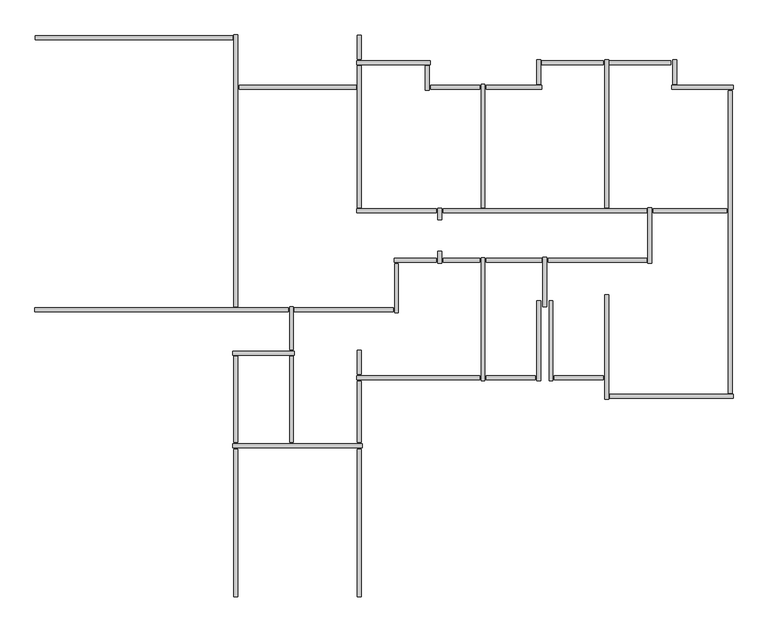
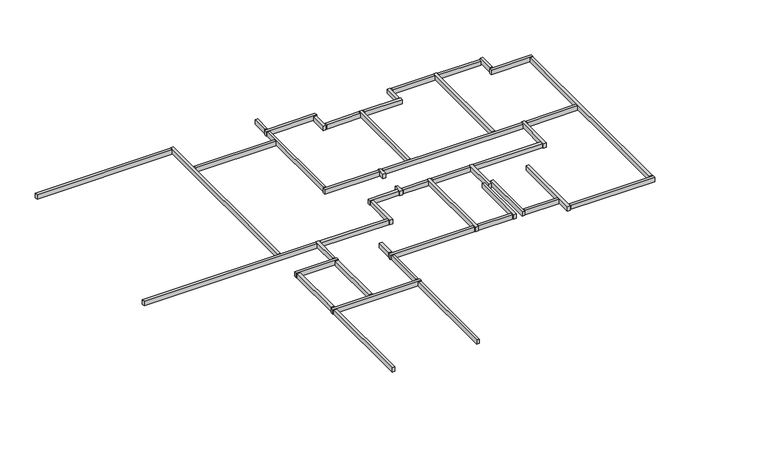
"""IFC4 building model written with IfcOpenShell, lengths in millimetres: beam geometry, Graute viga de respaldo5 : Graute viga de respaldo."""

import ifcopenshell
import ifcopenshell.guid

model = None  # the IFC model being written
_history = None  # IfcOwnerHistory: only IFC2X3 demands one
_inside = {}  # id of a spatial element -> (the spatial element, [elements in it])
_under = {}  # id of a project, library or spatial element -> (it, [spatial elements below it])
_declared = {}  # id of a project -> (the project, [libraries it declares])
_typed = {}  # id of a type object -> (the type object, [elements of that type])
_made_of = {}  # id of a material, layer set ... -> (it, [elements and type objects made of it])


def new_model(schema):
    """Start an empty IFC model of exactly this schema.

    Asked for "IFC4X3", IfcOpenShell would pick the latest addendum, in which some entities
    have other attributes; the version numbers below select the first issue.
    IFC2X3 requires an IfcOwnerHistory on every rooted entity: one is made here for all.
    """
    global model, _history
    if schema == "IFC4X3":
        model = ifcopenshell.file(schema_version=(4, 3, 0, 0))
    else:
        model = ifcopenshell.file(schema=schema)
    _inside.clear()
    _under.clear()
    _declared.clear()
    _typed.clear()
    _made_of.clear()
    _history = None
    if model.schema == "IFC2X3":
        org = make("IfcOrganization", Name="unknown")
        user = make(
            "IfcPersonAndOrganization",
            ThePerson=make("IfcPerson", FamilyName="unknown"),
            TheOrganization=org,
        )
        app = make(
            "IfcApplication",
            ApplicationDeveloper=org,
            Version="unknown",
            ApplicationFullName="unknown",
            ApplicationIdentifier="unknown",
        )
        _history = make(
            "IfcOwnerHistory",
            OwningUser=user,
            OwningApplication=app,
            ChangeAction="ADDED",
            CreationDate=0,
        )
    return model


def make(cls, **values):
    """One entity of the class cls with the attributes given. An attribute that is None is left unset."""
    return model.create_entity(
        cls, **{name: value for name, value in values.items() if value is not None}
    )


def rooted(cls, **values):
    """An entity with a GlobalId (a new one), such as an element, a storey or a relation."""
    return make(cls, GlobalId=ifcopenshell.guid.new(), OwnerHistory=_history, **values)


def si_unit(unit_type, name, prefix=None):
    """IfcSIUnit, for example si_unit("LENGTHUNIT", "METRE", prefix="MILLI")."""
    return make("IfcSIUnit", UnitType=unit_type, Prefix=prefix, Name=name)


def assignment(units):
    """IfcUnitAssignment: the units of a project."""
    return None if units is None else make("IfcUnitAssignment", Units=units)


def point(xyz):
    """IfcCartesianPoint."""
    return None if xyz is None else make("IfcCartesianPoint", Coordinates=xyz)


def direction(xyz):
    """IfcDirection."""
    return None if xyz is None else make("IfcDirection", DirectionRatios=xyz)


def frame(location, z_axis=None, x_axis=None):
    """IfcAxis2Placement3D, a coordinate frame: its origin and axes. An axis left out is left unset."""
    return make(
        "IfcAxis2Placement3D",
        Location=point(location),
        Axis=direction(z_axis),
        RefDirection=direction(x_axis),
    )


def origin():
    """The frame at (0, 0, 0) with its axes left unset."""
    return frame((0.0, 0.0, 0.0))


def place(relative_to, where):
    """IfcLocalPlacement: puts the frame where relative to a parent placement (None: the world)."""
    return make(
        "IfcLocalPlacement", PlacementRelTo=relative_to, RelativePlacement=where
    )


def context(
    kind, dimensions, precision=None, world=None, true_north=None, identifier=None
):
    """IfcGeometricRepresentationContext, for example the 3D "Model" context."""
    return make(
        "IfcGeometricRepresentationContext",
        ContextIdentifier=identifier,
        ContextType=kind,
        CoordinateSpaceDimension=dimensions,
        Precision=precision,
        WorldCoordinateSystem=world,
        TrueNorth=true_north,
    )


def project(units=None, contexts=None):
    """IfcProject with its units and contexts."""
    return rooted(
        "IfcProject",
        Name="project",
        RepresentationContexts=contexts,
        UnitsInContext=assignment(units),
    )


def spatial(cls, under=None, at=None, **own):
    """A site, building, storey or space (cls), placed at a placement, below another one or the project."""
    s = rooted(cls, ObjectPlacement=at, **own)
    if under is not None:
        _under.setdefault(under.id(), (under, []))[1].append(s)
    return s


def polyline(points):
    """IfcPolyline through the points."""
    return make("IfcPolyline", Points=[point(p) for p in points])


def outline(outer, holes=None, kind="AREA"):
    """IfcArbitraryClosedProfileDef: a profile drawn as a closed curve; with holes, ...WithVoids."""
    if holes is None:
        return make("IfcArbitraryClosedProfileDef", ProfileType=kind, OuterCurve=outer)
    return make(
        "IfcArbitraryProfileDefWithVoids",
        ProfileType=kind,
        OuterCurve=outer,
        InnerCurves=holes,
    )


def extrude(swept, where, along, depth):
    """IfcExtrudedAreaSolid: the profile swept, set in the frame where, extruded along a direction by depth."""
    return make(
        "IfcExtrudedAreaSolid",
        SweptArea=swept,
        Position=where,
        ExtrudedDirection=direction(along),
        Depth=depth,
    )


def shape(context_of_items, identifier, shape_type, items):
    """IfcShapeRepresentation: the items that make up one representation, for example the "Body"."""
    return make(
        "IfcShapeRepresentation",
        ContextOfItems=context_of_items,
        RepresentationIdentifier=identifier,
        RepresentationType=shape_type,
        Items=items,
    )


def source(mapping_origin, context_of_items, identifier, shape_type, items):
    """IfcRepresentationMap: a shape defined once, which mapped items show again and again."""
    return make(
        "IfcRepresentationMap",
        MappingOrigin=mapping_origin,
        MappedRepresentation=shape(context_of_items, identifier, shape_type, items),
    )


def transform(
    local_origin,
    x_axis=None,
    y_axis=None,
    z_axis=None,
    scale=None,
    scale2=None,
    scale3=None,
    uniform=True,
):
    """IfcCartesianTransformationOperator3D, or its non-uniform kind. x_axis, y_axis, z_axis: its Axis1, 2, 3."""
    if uniform:
        return make(
            "IfcCartesianTransformationOperator3D",
            Axis1=direction(x_axis),
            Axis2=direction(y_axis),
            LocalOrigin=point(local_origin),
            Scale=scale,
            Axis3=direction(z_axis),
        )
    return make(
        "IfcCartesianTransformationOperator3DnonUniform",
        Axis1=direction(x_axis),
        Axis2=direction(y_axis),
        LocalOrigin=point(local_origin),
        Scale=scale,
        Axis3=direction(z_axis),
        Scale2=scale2,
        Scale3=scale3,
    )


def mapped(mapping_source, mapping_target):
    """IfcMappedItem: shows the shape of a source again, moved by a transform."""
    return make(
        "IfcMappedItem", MappingSource=mapping_source, MappingTarget=mapping_target
    )


def made_of(thing, what):
    """Note that an element or type object is made of a material, layer set ...; save() writes the relation."""
    if what is not None:
        _made_of.setdefault(what.id(), (what, []))[1].append(thing)
    return thing


def element(
    cls,
    number,
    at=None,
    inside=None,
    cuts=None,
    type_object=None,
    material=None,
    context=None,
    identifier="Body",
    shape_type=None,
    held_by="IfcProductDefinitionShape",
    body=None,
    shapes=None,
    **own,
):
    """One element of the class cls, such as IfcWall. Its Tag is "e" and its number.

    at: its placement. inside: the storey or other place that contains it. cuts: it is an
    opening in that element (IfcRelVoidsElement). A single representation is given by context,
    identifier, shape_type and body (its items); several are given by shapes. held_by: the class
    of the entity that holds the representations. save() writes the other relations.
    """
    e = rooted(cls, Tag="e%d" % number, ObjectPlacement=at, **own)
    if body is not None:
        shapes = [shape(context, identifier, shape_type, body)]
    if shapes is not None:
        e.Representation = make(held_by, Representations=shapes)
    if inside is not None:
        _inside.setdefault(inside.id(), (inside, []))[1].append(e)
    if cuts is not None:
        rooted(
            "IfcRelVoidsElement", RelatingBuildingElement=cuts, RelatedOpeningElement=e
        )
    if type_object is not None:
        _typed.setdefault(type_object.id(), (type_object, []))[1].append(e)
    return made_of(e, material)


def aggregate(whole, parts):
    """IfcRelAggregates: a whole, such as a stair, and the parts it consists of."""
    return rooted("IfcRelAggregates", RelatingObject=whole, RelatedObjects=parts)


def save(model, path):
    """Write the relations noted so far, then the file.

    IfcRelAggregates (storeys below a building ...), IfcRelContainedInSpatialStructure (elements
    in a storey), IfcRelDefinesByType, IfcRelAssociatesMaterial and IfcRelDeclares: one each for
    every whole, place, type object, material and project.
    """
    for whole, parts in _under.values():
        aggregate(whole, parts)
    for where, things in _inside.values():
        rooted(
            "IfcRelContainedInSpatialStructure",
            RelatedElements=things,
            RelatingStructure=where,
        )
    for kind, things in _typed.values():
        rooted("IfcRelDefinesByType", RelatedObjects=things, RelatingType=kind)
    for what, things in _made_of.values():
        rooted("IfcRelAssociatesMaterial", RelatedObjects=things, RelatingMaterial=what)
    for by, libraries in _declared.values():
        rooted("IfcRelDeclares", RelatingContext=by, RelatedDefinitions=libraries)
    model.write(path)


def beam_6c566d9e(model_context):
    return source(origin(), model_context, "Body", "SweptSolid", [
        extrude(outline(polyline([(-62804.9587292, 72814.9577736), (-62804.9587292, 72720.9577736), (-67594.9587292, 72720.9577736), (-67594.9587292, 72814.9577736), (-62804.9587292, 72814.9577736)])), frame((0.0, 0.0, 5632.9999999), z_axis=(0.0, 0.0, 1.0), x_axis=(1.0, 0.0, 0.0)), (0.0, 0.0, 1.0), 167.0),
        extrude(outline(polyline([(-59771.9587292, 62785.4278788), (-59677.9587292, 62785.4278788), (-59677.9587292, 59195.4278788), (-59771.9587292, 59195.4278788), (-59771.9587292, 62785.4278788)])), frame((0.0, 0.0, 5632.9999999), z_axis=(0.0, 0.0, 1.0), x_axis=(1.0, 0.0, 0.0)), (0.0, 0.0, 1.0), 167.0),
        extrude(outline(polyline([(-62771.9587292, 62785.4278788), (-62677.9587292, 62785.4278788), (-62677.9587292, 59195.4278788), (-62771.9587292, 59195.4278788), (-62771.9587292, 62785.4278788)])), frame((0.0, 0.0, 5632.9999999), z_axis=(0.0, 0.0, 1.0), x_axis=(1.0, 0.0, 0.0)), (0.0, 0.0, 1.0), 167.0),
        extrude(outline(polyline([(-54994.9587292, 64468.4278788), (-54994.9587292, 64562.4278788), (-53804.9587292, 64562.4278788), (-53804.9587292, 64468.4278788), (-54994.9587292, 64468.4278788)])), frame((0.0, 0.0, 5632.9999999), z_axis=(0.0, 0.0, 1.0), x_axis=(1.0, 0.0, 0.0)), (0.0, 0.0, 1.0), 167.0),
        extrude(outline(polyline([(-56644.9587292, 64468.4278788), (-56644.9587292, 64562.4278788), (-55454.9587292, 64562.4278788), (-55454.9587292, 64468.4278788), (-56644.9587292, 64468.4278788)])), frame((0.0, 0.0, 5632.9999999), z_axis=(0.0, 0.0, 1.0), x_axis=(1.0, 0.0, 0.0)), (0.0, 0.0, 1.0), 167.0),
        extrude(outline(polyline([(-52594.9587292, 68518.4278788), (-52594.9587292, 68612.4278788), (-50804.9587292, 68612.4278788), (-50804.9587292, 68518.4278788), (-52594.9587292, 68518.4278788)])), frame((0.0, 0.0, 5632.9999999), z_axis=(0.0, 0.0, 1.0), x_axis=(1.0, 0.0, 0.0)), (0.0, 0.0, 1.0), 167.0),
        extrude(outline(polyline([(-57994.9587292, 71518.4278788), (-57994.9587292, 71612.4278788), (-56804.9587292, 71612.4278788), (-56804.9587292, 71518.4278788), (-57994.9587292, 71518.4278788)])), frame((0.0, 0.0, 5632.9999999), z_axis=(0.0, 0.0, 1.0), x_axis=(1.0, 0.0, 0.0)), (0.0, 0.0, 1.0), 167.0),
        extrude(outline(polyline([(-58027.9587292, 71495.4278788), (-58121.9587292, 71495.4278788), (-58121.9587292, 72085.4278788), (-58027.9587292, 72085.4278788), (-58027.9587292, 71495.4278788)])), frame((0.0, 0.0, 5632.9999999), z_axis=(0.0, 0.0, 1.0), x_axis=(1.0, 0.0, 0.0)), (0.0, 0.0, 1.0), 167.0),
        extrude(outline(polyline([(-59794.9587292, 72118.4278788), (-59794.9587292, 72212.4278788), (-58004.9587292, 72212.4278788), (-58004.9587292, 72118.4278788), (-59794.9587292, 72118.4278788)])), frame((0.0, 0.0, 5632.9999999), z_axis=(0.0, 0.0, 1.0), x_axis=(1.0, 0.0, 0.0)), (0.0, 0.0, 1.0), 167.0),
        extrude(outline(polyline([(-57821.9587292, 68635.4278788), (-57727.9587292, 68635.4278788), (-57727.9587292, 68345.4278788), (-57821.9587292, 68345.4278788), (-57821.9587292, 68635.4278788)])), frame((0.0, 0.0, 5632.9999999), z_axis=(0.0, 0.0, 1.0), x_axis=(1.0, 0.0, 0.0)), (0.0, 0.0, 1.0), 167.0),
        extrude(outline(polyline([(-55144.9587292, 67318.4278788), (-55144.9587292, 67412.4278788), (-52754.9587292, 67412.4278788), (-52754.9587292, 67318.4278788), (-55144.9587292, 67318.4278788)])), frame((0.0, 0.0, 5632.9999999), z_axis=(0.0, 0.0, 1.0), x_axis=(1.0, 0.0, 0.0)), (0.0, 0.0, 1.0), 167.0),
        extrude(outline(polyline([(-56644.9587292, 67318.4278788), (-56644.9587292, 67412.4278788), (-55304.9587292, 67412.4278788), (-55304.9587292, 67318.4278788), (-56644.9587292, 67318.4278788)])), frame((0.0, 0.0, 5632.9999999), z_axis=(0.0, 0.0, 1.0), x_axis=(1.0, 0.0, 0.0)), (0.0, 0.0, 1.0), 167.0),
        extrude(outline(polyline([(-57694.9587292, 67318.4278788), (-57694.9587292, 67412.4278788), (-56804.9587292, 67412.4278788), (-56804.9587292, 67318.4278788), (-57694.9587292, 67318.4278788)])), frame((0.0, 0.0, 5632.9999999), z_axis=(0.0, 0.0, 1.0), x_axis=(1.0, 0.0, 0.0)), (0.0, 0.0, 1.0), 167.0),
        extrude(outline(polyline([(-57821.9587292, 67585.4278788), (-57727.9587292, 67585.4278788), (-57727.9587292, 67295.4278788), (-57821.9587292, 67295.4278788), (-57821.9587292, 67585.4278788)])), frame((0.0, 0.0, 5632.9999999), z_axis=(0.0, 0.0, 1.0), x_axis=(1.0, 0.0, 0.0)), (0.0, 0.0, 1.0), 167.0),
        extrude(outline(polyline([(-58884.9587292, 67318.4278788), (-58884.9587292, 67412.4278788), (-57854.9587292, 67412.4278788), (-57854.9587292, 67318.4278788), (-58884.9587292, 67318.4278788)])), frame((0.0, 0.0, 5632.9999999), z_axis=(0.0, 0.0, 1.0), x_axis=(1.0, 0.0, 0.0)), (0.0, 0.0, 1.0), 167.0),
        extrude(outline(polyline([(-58777.9587292, 66095.4278788), (-58871.9587292, 66095.4278788), (-58871.9587292, 67285.4278788), (-58777.9587292, 67285.4278788), (-58777.9587292, 66095.4278788)])), frame((0.0, 0.0, 5632.9999999), z_axis=(0.0, 0.0, 1.0), x_axis=(1.0, 0.0, 0.0)), (0.0, 0.0, 1.0), 167.0),
        extrude(outline(polyline([(-61304.9587292, 66118.4278788), (-61304.9587292, 66212.4278788), (-58904.9587292, 66212.4278788), (-58904.9587292, 66118.4278788), (-61304.9587292, 66118.4278788)])), frame((0.0, 0.0, 5632.9999999), z_axis=(0.0, 0.0, 1.0), x_axis=(1.0, 0.0, 0.0)), (0.0, 0.0, 1.0), 167.0),
        extrude(outline(polyline([(-56771.9587292, 67430.4278788), (-56677.9587292, 67430.4278788), (-56677.9587292, 64445.4278788), (-56771.9587292, 64445.4278788), (-56771.9587292, 67430.4278788)])), frame((0.0, 0.0, 5632.9999999), z_axis=(0.0, 0.0, 1.0), x_axis=(1.0, 0.0, 0.0)), (0.0, 0.0, 1.0), 167.0),
        extrude(outline(polyline([(-59794.9587292, 64468.4278788), (-59794.9587292, 64562.4278788), (-56804.9587292, 64562.4278788), (-56804.9587292, 64468.4278788), (-59794.9587292, 64468.4278788)])), frame((0.0, 0.0, 5632.9999999), z_axis=(0.0, 0.0, 1.0), x_axis=(1.0, 0.0, 0.0)), (0.0, 0.0, 1.0), 167.0),
        extrude(outline(polyline([(-59771.9587292, 65185.4278788), (-59677.9587292, 65185.4278788), (-59677.9587292, 64595.4278788), (-59771.9587292, 64595.4278788), (-59771.9587292, 65185.4278788)])), frame((0.0, 0.0, 5632.9999999), z_axis=(0.0, 0.0, 1.0), x_axis=(1.0, 0.0, 0.0)), (0.0, 0.0, 1.0), 167.0),
        extrude(outline(polyline([(-59677.9587292, 62945.4278788), (-59771.9587292, 62945.4278788), (-59771.9587292, 64435.4278788), (-59677.9587292, 64435.4278788), (-59677.9587292, 62945.4278788)])), frame((0.0, 0.0, 5632.9999999), z_axis=(0.0, 0.0, 1.0), x_axis=(1.0, 0.0, 0.0)), (0.0, 0.0, 1.0), 167.0),
        extrude(outline(polyline([(-62677.9587292, 62945.4278788), (-62771.9587292, 62945.4278788), (-62771.9587292, 65035.4278788), (-62677.9587292, 65035.4278788), (-62677.9587292, 62945.4278788)])), frame((0.0, 0.0, 5632.9999999), z_axis=(0.0, 0.0, 1.0), x_axis=(1.0, 0.0, 0.0)), (0.0, 0.0, 1.0), 167.0),
        extrude(outline(polyline([(-61327.9587292, 62945.4278788), (-61421.9587292, 62945.4278788), (-61421.9587292, 65035.4278788), (-61327.9587292, 65035.4278788), (-61327.9587292, 62945.4278788)])), frame((0.0, 0.0, 5632.9999999), z_axis=(0.0, 0.0, 1.0), x_axis=(1.0, 0.0, 0.0)), (0.0, 0.0, 1.0), 167.0),
        extrude(outline(polyline([(-61421.9587292, 66235.4278788), (-61327.9587292, 66235.4278788), (-61327.9587292, 65195.4278788), (-61421.9587292, 65195.4278788), (-61421.9587292, 66235.4278788)])), frame((0.0, 0.0, 5632.9999999), z_axis=(0.0, 0.0, 1.0), x_axis=(1.0, 0.0, 0.0)), (0.0, 0.0, 1.0), 167.0),
        extrude(outline(polyline([(-62644.9587292, 71518.4278788), (-62644.9587292, 71612.4278788), (-59804.9587292, 71612.4278788), (-59804.9587292, 71518.4278788), (-62644.9587292, 71518.4278788)])), frame((0.0, 0.0, 5632.9999999), z_axis=(0.0, 0.0, 1.0), x_axis=(1.0, 0.0, 0.0)), (0.0, 0.0, 1.0), 167.0),
        extrude(outline(polyline([(-59677.9587292, 68645.4278788), (-59771.9587292, 68645.4278788), (-59771.9587292, 72085.4278788), (-59677.9587292, 72085.4278788), (-59677.9587292, 68645.4278788)])), frame((0.0, 0.0, 5632.9999999), z_axis=(0.0, 0.0, 1.0), x_axis=(1.0, 0.0, 0.0)), (0.0, 0.0, 1.0), 167.0),
        extrude(outline(polyline([(-59794.9587292, 68518.4278788), (-59794.9587292, 68612.4278788), (-57854.9587292, 68612.4278788), (-57854.9587292, 68518.4278788), (-59794.9587292, 68518.4278788)])), frame((0.0, 0.0, 5632.9999999), z_axis=(0.0, 0.0, 1.0), x_axis=(1.0, 0.0, 0.0)), (0.0, 0.0, 1.0), 167.0),
        extrude(outline(polyline([(-57694.9587292, 68518.4278788), (-57694.9587292, 68612.4278788), (-52754.9587292, 68612.4278788), (-52754.9587292, 68518.4278788), (-57694.9587292, 68518.4278788)])), frame((0.0, 0.0, 5632.9999999), z_axis=(0.0, 0.0, 1.0), x_axis=(1.0, 0.0, 0.0)), (0.0, 0.0, 1.0), 167.0),
        extrude(outline(polyline([(-56771.9587292, 71635.4278788), (-56677.9587292, 71635.4278788), (-56677.9587292, 68645.4278788), (-56771.9587292, 68645.4278788), (-56771.9587292, 71635.4278788)])), frame((0.0, 0.0, 5632.9999999), z_axis=(0.0, 0.0, 1.0), x_axis=(1.0, 0.0, 0.0)), (0.0, 0.0, 1.0), 167.0),
        extrude(outline(polyline([(-55304.9587292, 71612.4278788), (-55304.9587292, 71518.4278788), (-56644.9587292, 71518.4278788), (-56644.9587292, 71612.4278788), (-55304.9587292, 71612.4278788)])), frame((0.0, 0.0, 5632.9999999), z_axis=(0.0, 0.0, 1.0), x_axis=(1.0, 0.0, 0.0)), (0.0, 0.0, 1.0), 167.0),
        extrude(outline(polyline([(-55421.9587292, 72235.4278788), (-55327.9587292, 72235.4278788), (-55327.9587292, 71645.4278788), (-55421.9587292, 71645.4278788), (-55421.9587292, 72235.4278788)])), frame((0.0, 0.0, 5632.9999999), z_axis=(0.0, 0.0, 1.0), x_axis=(1.0, 0.0, 0.0)), (0.0, 0.0, 1.0), 167.0),
        extrude(outline(polyline([(-55294.9587292, 72118.4278788), (-55294.9587292, 72212.4278788), (-53804.9587292, 72212.4278788), (-53804.9587292, 72118.4278788), (-55294.9587292, 72118.4278788)])), frame((0.0, 0.0, 5632.9999999), z_axis=(0.0, 0.0, 1.0), x_axis=(1.0, 0.0, 0.0)), (0.0, 0.0, 1.0), 167.0),
        extrude(outline(polyline([(-52165.9809043, 72212.4278788), (-52165.9809043, 72117.4278788), (-53654.9587292, 72117.4278788), (-53654.9587292, 72212.4278788), (-52165.9809043, 72212.4278788)])), frame((0.0, 0.0, 5617.1856208), z_axis=(0.0, 0.0, 1.0), x_axis=(1.0, 0.0, 0.0)), (0.0, 0.0, 1.0), 165.0),
        extrude(outline(polyline([(-50677.9587292, 64145.4278788), (-50771.9587292, 64145.4278788), (-50771.9587292, 71485.4278788), (-50677.9587292, 71485.4278788), (-50677.9587292, 64145.4278788)])), frame((0.0, 0.0, 5632.9999999), z_axis=(0.0, 0.0, 1.0), x_axis=(1.0, 0.0, 0.0)), (0.0, 0.0, 1.0), 167.0),
        extrude(outline(polyline([(-52627.9587292, 67295.4278788), (-52721.9587292, 67295.4278788), (-52721.9587292, 68640.7810915), (-52627.9587292, 68640.7810915), (-52627.9587292, 67295.4278788)])), frame((0.0, 0.0, 5632.9999999), z_axis=(0.0, 0.0, 1.0), x_axis=(1.0, 0.0, 0.0)), (0.0, 0.0, 1.0), 167.0),
        extrude(outline(polyline([(-55177.9587292, 66245.4278788), (-55271.9587292, 66245.4278788), (-55271.9587292, 67435.4278788), (-55177.9587292, 67435.4278788), (-55177.9587292, 66245.4278788)])), frame((0.0, 0.0, 5632.9999999), z_axis=(0.0, 0.0, 1.0), x_axis=(1.0, 0.0, 0.0)), (0.0, 0.0, 1.0), 167.0),
        extrude(outline(polyline([(-55027.9587292, 64445.4278788), (-55121.9587292, 64445.4278788), (-55121.9587292, 66385.4278788), (-55027.9587292, 66385.4278788), (-55027.9587292, 64445.4278788)])), frame((0.0, 0.0, 5632.9999999), z_axis=(0.0, 0.0, 1.0), x_axis=(1.0, 0.0, 0.0)), (0.0, 0.0, 1.0), 167.0),
        extrude(outline(polyline([(-55327.9587292, 64445.4278788), (-55421.9587292, 64445.4278788), (-55421.9587292, 66385.4278788), (-55327.9587292, 66385.4278788), (-55327.9587292, 64445.4278788)])), frame((0.0, 0.0, 5632.9999999), z_axis=(0.0, 0.0, 1.0), x_axis=(1.0, 0.0, 0.0)), (0.0, 0.0, 1.0), 167.0),
        extrude(outline(polyline([(-53677.9587292, 63995.4278788), (-53771.9587292, 63995.4278788), (-53771.9587292, 66535.4278788), (-53677.9587292, 66535.4278788), (-53677.9587292, 63995.4278788)])), frame((0.0, 0.0, 5632.9999999), z_axis=(0.0, 0.0, 1.0), x_axis=(1.0, 0.0, 0.0)), (0.0, 0.0, 1.0), 167.0),
        extrude(outline(polyline([(-50654.9587292, 64112.4278788), (-50654.9587292, 64018.4278788), (-53644.9587292, 64018.4278788), (-53644.9587292, 64112.4278788), (-50654.9587292, 64112.4278788)])), frame((0.0, 0.0, 5632.9999999), z_axis=(0.0, 0.0, 1.0), x_axis=(1.0, 0.0, 0.0)), (0.0, 0.0, 1.0), 167.0),
        extrude(outline(polyline([(-52121.9587292, 72235.4278788), (-52027.9587292, 72235.4278788), (-52027.9587292, 71645.4278788), (-52121.9587292, 71645.4278788), (-52121.9587292, 72235.4278788)])), frame((0.0, 0.0, 5632.9999999), z_axis=(0.0, 0.0, 1.0), x_axis=(1.0, 0.0, 0.0)), (0.0, 0.0, 1.0), 167.0),
        extrude(outline(polyline([(-52144.9587292, 71518.4278788), (-52144.9587292, 71612.4278788), (-50654.9587292, 71612.4278788), (-50654.9587292, 71518.4278788), (-52144.9587292, 71518.4278788)])), frame((0.0, 0.0, 5632.9999999), z_axis=(0.0, 0.0, 1.0), x_axis=(1.0, 0.0, 0.0)), (0.0, 0.0, 1.0), 167.0),
        extrude(outline(polyline([(-53771.9587292, 72235.4278788), (-53677.9587292, 72235.4278788), (-53677.9587292, 68645.4278788), (-53771.9587292, 68645.4278788), (-53771.9587292, 72235.4278788)])), frame((0.0, 0.0, 5632.9999999), z_axis=(0.0, 0.0, 1.0), x_axis=(1.0, 0.0, 0.0)), (0.0, 0.0, 1.0), 167.0),
        extrude(outline(polyline([(-59771.9587292, 72835.4278788), (-59677.9587292, 72835.4278788), (-59677.9587292, 72245.4278788), (-59771.9587292, 72245.4278788), (-59771.9587292, 72835.4278788)])), frame((0.0, 0.0, 5632.9999999), z_axis=(0.0, 0.0, 1.0), x_axis=(1.0, 0.0, 0.0)), (0.0, 0.0, 1.0), 167.0),
        extrude(outline(polyline([(-62794.9587292, 65068.4278788), (-62794.9587292, 65162.4278788), (-61304.9587292, 65162.4278788), (-61304.9587292, 65068.4278788), (-62794.9587292, 65068.4278788)])), frame((0.0, 0.0, 5632.9999999), z_axis=(0.0, 0.0, 1.0), x_axis=(1.0, 0.0, 0.0)), (0.0, 0.0, 1.0), 167.0),
        extrude(outline(polyline([(-62794.9587292, 62818.4278788), (-62794.9587292, 62912.4278788), (-59654.9587292, 62912.4278788), (-59654.9587292, 62818.4278788), (-62794.9587292, 62818.4278788)])), frame((0.0, 0.0, 5632.9999999), z_axis=(0.0, 0.0, 1.0), x_axis=(1.0, 0.0, 0.0)), (0.0, 0.0, 1.0), 167.0),
        extrude(outline(polyline([(-67601.7587292, 66118.4278788), (-67601.7587292, 66212.4278788), (-61454.9587292, 66212.4278788), (-61454.9587292, 66118.4278788), (-67601.7587292, 66118.4278788)])), frame((0.0, 0.0, 5632.9999999), z_axis=(0.0, 0.0, 1.0), x_axis=(1.0, 0.0, 0.0)), (0.0, 0.0, 1.0), 167.0),
        extrude(outline(polyline([(-62771.9587292, 72837.9577736), (-62677.9587292, 72837.9577736), (-62677.9587292, 66245.4278788), (-62771.9587292, 66245.4278788), (-62771.9587292, 72837.9577736)])), frame((0.0, 0.0, 5632.9999999), z_axis=(0.0, 0.0, 1.0), x_axis=(1.0, 0.0, 0.0)), (0.0, 0.0, 1.0), 167.0),
    ])


if __name__ == "__main__":
    model = new_model("IFC4")
    model_context = context("Model", 3, world=origin())
    ifc_project = project(units=[si_unit("LENGTHUNIT", "METRE", prefix="MILLI")], contexts=[model_context])
    site = spatial("IfcSite", under=ifc_project)
    building = spatial("IfcBuilding", under=site)
    placement = place(None, origin())
    beam_shape = beam_6c566d9e(model_context)
    element("IfcBeam", 1, ObjectType="Graute viga de respaldo5 : Graute viga de respaldo", at=placement, inside=building, context=model_context, shape_type="MappedRepresentation", body=[
        mapped(beam_shape, transform((0.0, 0.0, 0.0), x_axis=(1.0, 0.0, 0.0), y_axis=(0.0, 1.0, 0.0), z_axis=(0.0, 0.0, 1.0))),
    ])
    save(model, "model.ifc")

# Revit data of these elements
# Element 1 (IfcBeam, "Graute viga de respaldo5 : Graute viga de respaldo")
#   Materials on its faces: "Concreto, Faixa de areia/cimento"
# Materials
#   "Concreto, Faixa de areia/cimento": class "Concreto", colour RGB 127 127 127, transparency 0, Description = "Revestimento de laje de concreto", Cost = 0
